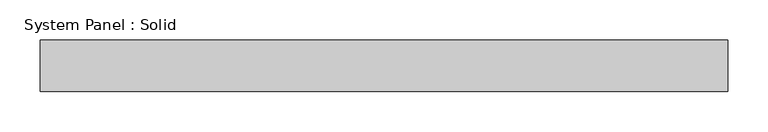
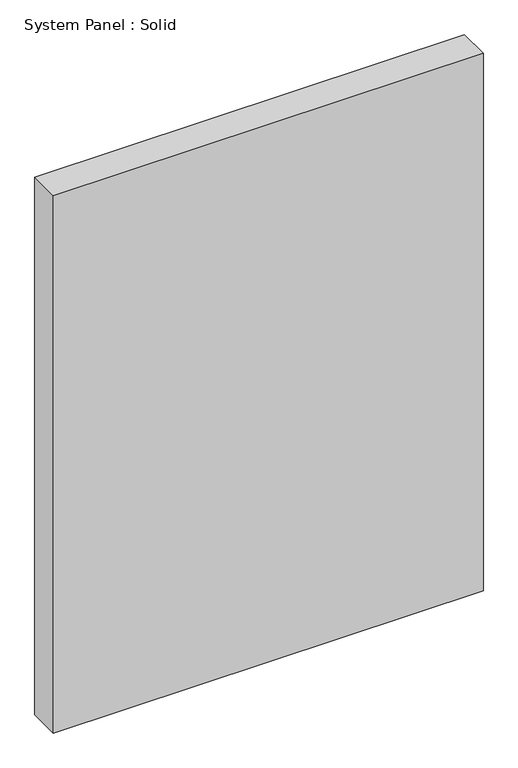
"""IFC4 building model written with IfcOpenShell, lengths in millimetres: plate geometry, System Panel : Solid."""

from ifc_helpers import new_model, si_unit, origin, origin_with_axes, place, context, project, spatial, polyline, outline, extrude, source, transform, mapped, element, save


def system_panel_solid_05eef404(model_context):
    return source(origin(), model_context, "Body", "SweptSolid", [
        extrude(outline(polyline([(425.45, -44.45), (-425.45, -44.45), (-425.45, 19.05), (425.45, 19.05), (425.45, -44.45)])), origin_with_axes(), (0.0, 0.0, 1.0), 1123.95),
    ])


if __name__ == "__main__":
    model = new_model("IFC4")
    model_context = context("Model", 3, world=origin())
    ifc_project = project(units=[si_unit("LENGTHUNIT", "METRE", prefix="MILLI")], contexts=[model_context])
    site = spatial("IfcSite", under=ifc_project)
    building = spatial("IfcBuilding", under=site)
    placement = place(None, origin())
    system_panel_solid_shape = system_panel_solid_05eef404(model_context)
    element("IfcPlate", 1, ObjectType="System Panel : Solid", at=placement, inside=building, context=model_context, shape_type="MappedRepresentation", body=[
        mapped(system_panel_solid_shape, transform((0.0, 0.0, 0.0), x_axis=(1.0, 0.0, 0.0), y_axis=(0.0, 1.0, 0.0), z_axis=(0.0, 0.0, 1.0))),
    ])
    save(model, "model.ifc")

# Revit data of these elements
# Type "System Panel : Solid"
#   Construction Type Id = "MDOOR"
#   Analytic Construction = "Metal"
#   Visual Light Transmittance = 0
#   Solar Heat Gain Coefficient = 0
#   Heat Transfer Coefficient (U) = 0.651978 BTU/(h·ft²·°F)
#   Define Thermal Properties by = 1
# Element 1 (IfcPlate, "System Panel : Solid")
#   Materials on its faces: "Default"
# Materials
#   "Default": class "Miscellaneous", colour RGB 127 127 127, transparency 0, Cost = 0
